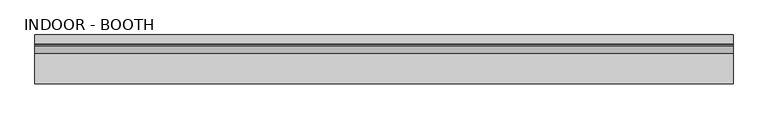
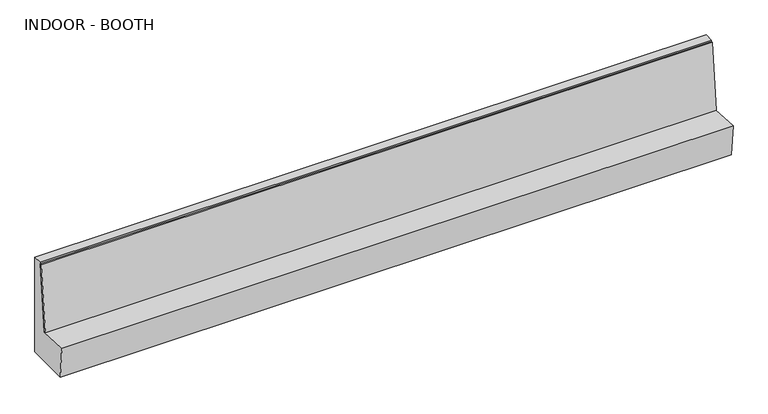
"""IFC4 building model written with IfcOpenShell, lengths in millimetres: furniture geometry, OD_CW_Booth : INDOOR - BOOTH."""

import ifcopenshell
import ifcopenshell.guid

model = None  # the IFC model being written
_history = None  # IfcOwnerHistory: only IFC2X3 demands one
_inside = {}  # id of a spatial element -> (the spatial element, [elements in it])
_under = {}  # id of a project, library or spatial element -> (it, [spatial elements below it])
_declared = {}  # id of a project -> (the project, [libraries it declares])
_typed = {}  # id of a type object -> (the type object, [elements of that type])
_made_of = {}  # id of a material, layer set ... -> (it, [elements and type objects made of it])


def new_model(schema):
    """Start an empty IFC model of exactly this schema.

    Asked for "IFC4X3", IfcOpenShell would pick the latest addendum, in which some entities
    have other attributes; the version numbers below select the first issue.
    IFC2X3 requires an IfcOwnerHistory on every rooted entity: one is made here for all.
    """
    global model, _history
    if schema == "IFC4X3":
        model = ifcopenshell.file(schema_version=(4, 3, 0, 0))
    else:
        model = ifcopenshell.file(schema=schema)
    _inside.clear()
    _under.clear()
    _declared.clear()
    _typed.clear()
    _made_of.clear()
    _history = None
    if model.schema == "IFC2X3":
        org = make("IfcOrganization", Name="unknown")
        user = make(
            "IfcPersonAndOrganization",
            ThePerson=make("IfcPerson", FamilyName="unknown"),
            TheOrganization=org,
        )
        app = make(
            "IfcApplication",
            ApplicationDeveloper=org,
            Version="unknown",
            ApplicationFullName="unknown",
            ApplicationIdentifier="unknown",
        )
        _history = make(
            "IfcOwnerHistory",
            OwningUser=user,
            OwningApplication=app,
            ChangeAction="ADDED",
            CreationDate=0,
        )
    return model


def make(cls, **values):
    """One entity of the class cls with the attributes given. An attribute that is None is left unset."""
    return model.create_entity(
        cls, **{name: value for name, value in values.items() if value is not None}
    )


def rooted(cls, **values):
    """An entity with a GlobalId (a new one), such as an element, a storey or a relation."""
    return make(cls, GlobalId=ifcopenshell.guid.new(), OwnerHistory=_history, **values)


def si_unit(unit_type, name, prefix=None):
    """IfcSIUnit, for example si_unit("LENGTHUNIT", "METRE", prefix="MILLI")."""
    return make("IfcSIUnit", UnitType=unit_type, Prefix=prefix, Name=name)


def assignment(units):
    """IfcUnitAssignment: the units of a project."""
    return None if units is None else make("IfcUnitAssignment", Units=units)


def point(xyz):
    """IfcCartesianPoint."""
    return None if xyz is None else make("IfcCartesianPoint", Coordinates=xyz)


def direction(xyz):
    """IfcDirection."""
    return None if xyz is None else make("IfcDirection", DirectionRatios=xyz)


def frame(location, z_axis=None, x_axis=None):
    """IfcAxis2Placement3D, a coordinate frame: its origin and axes. An axis left out is left unset."""
    return make(
        "IfcAxis2Placement3D",
        Location=point(location),
        Axis=direction(z_axis),
        RefDirection=direction(x_axis),
    )


def origin():
    """The frame at (0, 0, 0) with its axes left unset."""
    return frame((0.0, 0.0, 0.0))


def place(relative_to, where):
    """IfcLocalPlacement: puts the frame where relative to a parent placement (None: the world)."""
    return make(
        "IfcLocalPlacement", PlacementRelTo=relative_to, RelativePlacement=where
    )


def context(
    kind, dimensions, precision=None, world=None, true_north=None, identifier=None
):
    """IfcGeometricRepresentationContext, for example the 3D "Model" context."""
    return make(
        "IfcGeometricRepresentationContext",
        ContextIdentifier=identifier,
        ContextType=kind,
        CoordinateSpaceDimension=dimensions,
        Precision=precision,
        WorldCoordinateSystem=world,
        TrueNorth=true_north,
    )


def project(units=None, contexts=None):
    """IfcProject with its units and contexts."""
    return rooted(
        "IfcProject",
        Name="project",
        RepresentationContexts=contexts,
        UnitsInContext=assignment(units),
    )


def spatial(cls, under=None, at=None, **own):
    """A site, building, storey or space (cls), placed at a placement, below another one or the project."""
    s = rooted(cls, ObjectPlacement=at, **own)
    if under is not None:
        _under.setdefault(under.id(), (under, []))[1].append(s)
    return s


def polyline(points):
    """IfcPolyline through the points."""
    return make("IfcPolyline", Points=[point(p) for p in points])


def outline(outer, holes=None, kind="AREA"):
    """IfcArbitraryClosedProfileDef: a profile drawn as a closed curve; with holes, ...WithVoids."""
    if holes is None:
        return make("IfcArbitraryClosedProfileDef", ProfileType=kind, OuterCurve=outer)
    return make(
        "IfcArbitraryProfileDefWithVoids",
        ProfileType=kind,
        OuterCurve=outer,
        InnerCurves=holes,
    )


def extrude(swept, where, along, depth):
    """IfcExtrudedAreaSolid: the profile swept, set in the frame where, extruded along a direction by depth."""
    return make(
        "IfcExtrudedAreaSolid",
        SweptArea=swept,
        Position=where,
        ExtrudedDirection=direction(along),
        Depth=depth,
    )


def shape(context_of_items, identifier, shape_type, items):
    """IfcShapeRepresentation: the items that make up one representation, for example the "Body"."""
    return make(
        "IfcShapeRepresentation",
        ContextOfItems=context_of_items,
        RepresentationIdentifier=identifier,
        RepresentationType=shape_type,
        Items=items,
    )


def source(mapping_origin, context_of_items, identifier, shape_type, items):
    """IfcRepresentationMap: a shape defined once, which mapped items show again and again."""
    return make(
        "IfcRepresentationMap",
        MappingOrigin=mapping_origin,
        MappedRepresentation=shape(context_of_items, identifier, shape_type, items),
    )


def transform(
    local_origin,
    x_axis=None,
    y_axis=None,
    z_axis=None,
    scale=None,
    scale2=None,
    scale3=None,
    uniform=True,
):
    """IfcCartesianTransformationOperator3D, or its non-uniform kind. x_axis, y_axis, z_axis: its Axis1, 2, 3."""
    if uniform:
        return make(
            "IfcCartesianTransformationOperator3D",
            Axis1=direction(x_axis),
            Axis2=direction(y_axis),
            LocalOrigin=point(local_origin),
            Scale=scale,
            Axis3=direction(z_axis),
        )
    return make(
        "IfcCartesianTransformationOperator3DnonUniform",
        Axis1=direction(x_axis),
        Axis2=direction(y_axis),
        LocalOrigin=point(local_origin),
        Scale=scale,
        Axis3=direction(z_axis),
        Scale2=scale2,
        Scale3=scale3,
    )


def mapped(mapping_source, mapping_target):
    """IfcMappedItem: shows the shape of a source again, moved by a transform."""
    return make(
        "IfcMappedItem", MappingSource=mapping_source, MappingTarget=mapping_target
    )


def made_of(thing, what):
    """Note that an element or type object is made of a material, layer set ...; save() writes the relation."""
    if what is not None:
        _made_of.setdefault(what.id(), (what, []))[1].append(thing)
    return thing


def element(
    cls,
    number,
    at=None,
    inside=None,
    cuts=None,
    type_object=None,
    material=None,
    context=None,
    identifier="Body",
    shape_type=None,
    held_by="IfcProductDefinitionShape",
    body=None,
    shapes=None,
    **own,
):
    """One element of the class cls, such as IfcWall. Its Tag is "e" and its number.

    at: its placement. inside: the storey or other place that contains it. cuts: it is an
    opening in that element (IfcRelVoidsElement). A single representation is given by context,
    identifier, shape_type and body (its items); several are given by shapes. held_by: the class
    of the entity that holds the representations. save() writes the other relations.
    """
    e = rooted(cls, Tag="e%d" % number, ObjectPlacement=at, **own)
    if body is not None:
        shapes = [shape(context, identifier, shape_type, body)]
    if shapes is not None:
        e.Representation = make(held_by, Representations=shapes)
    if inside is not None:
        _inside.setdefault(inside.id(), (inside, []))[1].append(e)
    if cuts is not None:
        rooted(
            "IfcRelVoidsElement", RelatingBuildingElement=cuts, RelatedOpeningElement=e
        )
    if type_object is not None:
        _typed.setdefault(type_object.id(), (type_object, []))[1].append(e)
    return made_of(e, material)


def aggregate(whole, parts):
    """IfcRelAggregates: a whole, such as a stair, and the parts it consists of."""
    return rooted("IfcRelAggregates", RelatingObject=whole, RelatedObjects=parts)


def save(model, path):
    """Write the relations noted so far, then the file.

    IfcRelAggregates (storeys below a building ...), IfcRelContainedInSpatialStructure (elements
    in a storey), IfcRelDefinesByType, IfcRelAssociatesMaterial and IfcRelDeclares: one each for
    every whole, place, type object, material and project.
    """
    for whole, parts in _under.values():
        aggregate(whole, parts)
    for where, things in _inside.values():
        rooted(
            "IfcRelContainedInSpatialStructure",
            RelatedElements=things,
            RelatingStructure=where,
        )
    for kind, things in _typed.values():
        rooted("IfcRelDefinesByType", RelatedObjects=things, RelatingType=kind)
    for what, things in _made_of.values():
        rooted("IfcRelAssociatesMaterial", RelatedObjects=things, RelatingMaterial=what)
    for by, libraries in _declared.values():
        rooted("IfcRelDeclares", RelatingContext=by, RelatedDefinitions=libraries)
    model.write(path)


def indoor_booth_53f0a2fe(model_context):
    return source(origin(), model_context, "Body", "SweptSolid", [
        extrude(outline(polyline([(0.0, 9357.0837874), (25.4, 9357.0837874), (25.4, 0.0), (0.0, 0.0), (0.0, 9357.0837874)])), frame((9375.8214923, 358.2049359, 438.8309433), z_axis=(0.0, 0.10452846326765197, 0.9945218953682735), x_axis=(0.0, 0.9945218953682735, -0.10452846326765197)), (0.0, 0.0, 1.0), 944.7333479),
        extrude(outline(polyline([(609.6, 1397.0), (609.6, 0.0), (-3.4100193, 0.0), (-43.0849153, 453.4861359), (382.9385128, 431.1591941), (484.4524721, 1397.0), (609.6, 1397.0)])), frame((18.7377049, 0.0, 0.0), z_axis=(1.0, 0.0, 0.0), x_axis=(0.0, 1.0, 0.0)), (0.0, 0.0, 1.0), 9357.0837874),
    ])


if __name__ == "__main__":
    model = new_model("IFC4")
    model_context = context("Model", 3, world=origin())
    ifc_project = project(units=[si_unit("LENGTHUNIT", "METRE", prefix="MILLI")], contexts=[model_context])
    site = spatial("IfcSite", under=ifc_project)
    building = spatial("IfcBuilding", under=site)
    placement = place(None, origin())
    indoor_booth_shape = indoor_booth_53f0a2fe(model_context)
    element("IfcFurniture", 1, ObjectType="OD_CW_Booth : INDOOR - BOOTH", at=placement, inside=building, context=model_context, shape_type="MappedRepresentation", body=[
        mapped(indoor_booth_shape, transform((0.0, 0.0, 0.0), x_axis=(1.0, 0.0, 0.0), y_axis=(0.0, 1.0, 0.0), z_axis=(0.0, 0.0, 1.0))),
    ])
    save(model, "model.ifc")

# Revit data of these elements
# Type "OD_CW_Booth : INDOOR - BOOTH"
#   Type Mark = "TYPE - INDOOR - BOOTH"
#   Width = 4' - 0"
#   OD_CW_Width [instance default] = 2' - 10"
#   OD_CW_Length [instance default] = 26' - 1 83/256"
#   OD_CW_Height [instance default] = 2' - 3"
#   Height = 3' - 0"
#   Depth = 2' - 0"
#   Seating Count [instance default] = 10
#   Seating Count [instance default] = 10
#   back = WOOD VENEER
#   OD_CW_Material_Front Panel [instance default] = none
#   OD_CW_Material_Body [instance default] = none
# Element 1 (IfcFurniture, "OD_CW_Booth : INDOOR - BOOTH")
#   OD_CW_Length = 30' - 8.38913"
#   Seating Count = 11
#   OD_CW_Material_Body = WOOD-OAKFIRE
#   Materials on its faces: "WOOD-OAKFIRE", "WOOD VENEER"
# Materials
#   "WOOD VENEER": class "Miscellaneous", colour RGB 164 164 164, transparency 0, Cost = 0
#   "WOOD-OAKFIRE": class "Wood", colour RGB 198 202 183, transparency 0, Description = "Generic wood", Cost = 0
